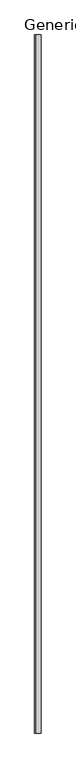
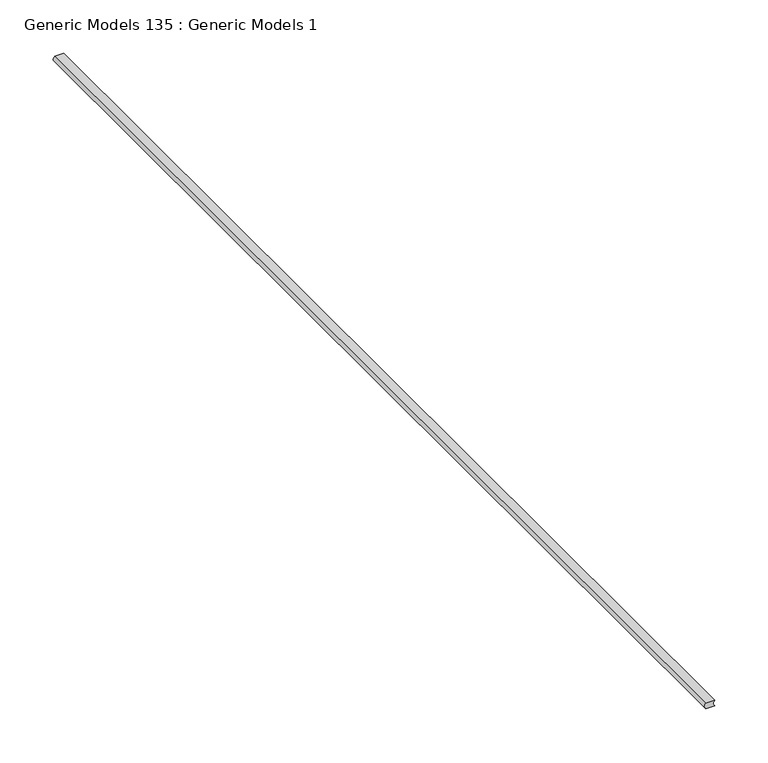
"""IFC4 building model written with IfcOpenShell, lengths in millimetres: proxy geometry, Generic Models 135 : Generic Models 1."""

import ifcopenshell
import ifcopenshell.guid

model = None  # the IFC model being written
_history = None  # IfcOwnerHistory: only IFC2X3 demands one
_inside = {}  # id of a spatial element -> (the spatial element, [elements in it])
_under = {}  # id of a project, library or spatial element -> (it, [spatial elements below it])
_declared = {}  # id of a project -> (the project, [libraries it declares])
_typed = {}  # id of a type object -> (the type object, [elements of that type])
_made_of = {}  # id of a material, layer set ... -> (it, [elements and type objects made of it])


def new_model(schema):
    """Start an empty IFC model of exactly this schema.

    Asked for "IFC4X3", IfcOpenShell would pick the latest addendum, in which some entities
    have other attributes; the version numbers below select the first issue.
    IFC2X3 requires an IfcOwnerHistory on every rooted entity: one is made here for all.
    """
    global model, _history
    if schema == "IFC4X3":
        model = ifcopenshell.file(schema_version=(4, 3, 0, 0))
    else:
        model = ifcopenshell.file(schema=schema)
    _inside.clear()
    _under.clear()
    _declared.clear()
    _typed.clear()
    _made_of.clear()
    _history = None
    if model.schema == "IFC2X3":
        org = make("IfcOrganization", Name="unknown")
        user = make(
            "IfcPersonAndOrganization",
            ThePerson=make("IfcPerson", FamilyName="unknown"),
            TheOrganization=org,
        )
        app = make(
            "IfcApplication",
            ApplicationDeveloper=org,
            Version="unknown",
            ApplicationFullName="unknown",
            ApplicationIdentifier="unknown",
        )
        _history = make(
            "IfcOwnerHistory",
            OwningUser=user,
            OwningApplication=app,
            ChangeAction="ADDED",
            CreationDate=0,
        )
    return model


def make(cls, **values):
    """One entity of the class cls with the attributes given. An attribute that is None is left unset."""
    return model.create_entity(
        cls, **{name: value for name, value in values.items() if value is not None}
    )


def rooted(cls, **values):
    """An entity with a GlobalId (a new one), such as an element, a storey or a relation."""
    return make(cls, GlobalId=ifcopenshell.guid.new(), OwnerHistory=_history, **values)


def si_unit(unit_type, name, prefix=None):
    """IfcSIUnit, for example si_unit("LENGTHUNIT", "METRE", prefix="MILLI")."""
    return make("IfcSIUnit", UnitType=unit_type, Prefix=prefix, Name=name)


def assignment(units):
    """IfcUnitAssignment: the units of a project."""
    return None if units is None else make("IfcUnitAssignment", Units=units)


def point(xyz):
    """IfcCartesianPoint."""
    return None if xyz is None else make("IfcCartesianPoint", Coordinates=xyz)


def direction(xyz):
    """IfcDirection."""
    return None if xyz is None else make("IfcDirection", DirectionRatios=xyz)


def frame(location, z_axis=None, x_axis=None):
    """IfcAxis2Placement3D, a coordinate frame: its origin and axes. An axis left out is left unset."""
    return make(
        "IfcAxis2Placement3D",
        Location=point(location),
        Axis=direction(z_axis),
        RefDirection=direction(x_axis),
    )


def frame_2d(location, x_axis=None):
    """IfcAxis2Placement2D, a coordinate frame in the plane: its origin and x axis."""
    return make(
        "IfcAxis2Placement2D", Location=point(location), RefDirection=direction(x_axis)
    )


def origin():
    """The frame at (0, 0, 0) with its axes left unset."""
    return frame((0.0, 0.0, 0.0))


def place(relative_to, where):
    """IfcLocalPlacement: puts the frame where relative to a parent placement (None: the world)."""
    return make(
        "IfcLocalPlacement", PlacementRelTo=relative_to, RelativePlacement=where
    )


def context(
    kind, dimensions, precision=None, world=None, true_north=None, identifier=None
):
    """IfcGeometricRepresentationContext, for example the 3D "Model" context."""
    return make(
        "IfcGeometricRepresentationContext",
        ContextIdentifier=identifier,
        ContextType=kind,
        CoordinateSpaceDimension=dimensions,
        Precision=precision,
        WorldCoordinateSystem=world,
        TrueNorth=true_north,
    )


def project(units=None, contexts=None):
    """IfcProject with its units and contexts."""
    return rooted(
        "IfcProject",
        Name="project",
        RepresentationContexts=contexts,
        UnitsInContext=assignment(units),
    )


def spatial(cls, under=None, at=None, **own):
    """A site, building, storey or space (cls), placed at a placement, below another one or the project."""
    s = rooted(cls, ObjectPlacement=at, **own)
    if under is not None:
        _under.setdefault(under.id(), (under, []))[1].append(s)
    return s


def polyline(points):
    """IfcPolyline through the points."""
    return make("IfcPolyline", Points=[point(p) for p in points])


def circle_curve(where, radius):
    """IfcCircle in the frame where."""
    return make("IfcCircle", Position=where, Radius=radius)


def trimmed(basis, trim1, trim2, sense, master):
    """IfcTrimmedCurve: the piece of a basis curve between two trims."""
    return make(
        "IfcTrimmedCurve",
        BasisCurve=basis,
        Trim1=trim1,
        Trim2=trim2,
        SenseAgreement=sense,
        MasterRepresentation=master,
    )


def segment(curve, same_sense, transition):
    """IfcCompositeCurveSegment."""
    return make(
        "IfcCompositeCurveSegment",
        Transition=transition,
        SameSense=same_sense,
        ParentCurve=curve,
    )


def composite_curve(segments, self_intersect=None):
    """IfcCompositeCurve: segments joined end to end."""
    return make("IfcCompositeCurve", Segments=segments, SelfIntersect=self_intersect)


def outline(outer, holes=None, kind="AREA"):
    """IfcArbitraryClosedProfileDef: a profile drawn as a closed curve; with holes, ...WithVoids."""
    if holes is None:
        return make("IfcArbitraryClosedProfileDef", ProfileType=kind, OuterCurve=outer)
    return make(
        "IfcArbitraryProfileDefWithVoids",
        ProfileType=kind,
        OuterCurve=outer,
        InnerCurves=holes,
    )


def extrude(swept, where, along, depth):
    """IfcExtrudedAreaSolid: the profile swept, set in the frame where, extruded along a direction by depth."""
    return make(
        "IfcExtrudedAreaSolid",
        SweptArea=swept,
        Position=where,
        ExtrudedDirection=direction(along),
        Depth=depth,
    )


def shape(context_of_items, identifier, shape_type, items):
    """IfcShapeRepresentation: the items that make up one representation, for example the "Body"."""
    return make(
        "IfcShapeRepresentation",
        ContextOfItems=context_of_items,
        RepresentationIdentifier=identifier,
        RepresentationType=shape_type,
        Items=items,
    )


def source(mapping_origin, context_of_items, identifier, shape_type, items):
    """IfcRepresentationMap: a shape defined once, which mapped items show again and again."""
    return make(
        "IfcRepresentationMap",
        MappingOrigin=mapping_origin,
        MappedRepresentation=shape(context_of_items, identifier, shape_type, items),
    )


def transform(
    local_origin,
    x_axis=None,
    y_axis=None,
    z_axis=None,
    scale=None,
    scale2=None,
    scale3=None,
    uniform=True,
):
    """IfcCartesianTransformationOperator3D, or its non-uniform kind. x_axis, y_axis, z_axis: its Axis1, 2, 3."""
    if uniform:
        return make(
            "IfcCartesianTransformationOperator3D",
            Axis1=direction(x_axis),
            Axis2=direction(y_axis),
            LocalOrigin=point(local_origin),
            Scale=scale,
            Axis3=direction(z_axis),
        )
    return make(
        "IfcCartesianTransformationOperator3DnonUniform",
        Axis1=direction(x_axis),
        Axis2=direction(y_axis),
        LocalOrigin=point(local_origin),
        Scale=scale,
        Axis3=direction(z_axis),
        Scale2=scale2,
        Scale3=scale3,
    )


def mapped(mapping_source, mapping_target):
    """IfcMappedItem: shows the shape of a source again, moved by a transform."""
    return make(
        "IfcMappedItem", MappingSource=mapping_source, MappingTarget=mapping_target
    )


def made_of(thing, what):
    """Note that an element or type object is made of a material, layer set ...; save() writes the relation."""
    if what is not None:
        _made_of.setdefault(what.id(), (what, []))[1].append(thing)
    return thing


def element(
    cls,
    number,
    at=None,
    inside=None,
    cuts=None,
    type_object=None,
    material=None,
    context=None,
    identifier="Body",
    shape_type=None,
    held_by="IfcProductDefinitionShape",
    body=None,
    shapes=None,
    **own,
):
    """One element of the class cls, such as IfcWall. Its Tag is "e" and its number.

    at: its placement. inside: the storey or other place that contains it. cuts: it is an
    opening in that element (IfcRelVoidsElement). A single representation is given by context,
    identifier, shape_type and body (its items); several are given by shapes. held_by: the class
    of the entity that holds the representations. save() writes the other relations.
    """
    e = rooted(cls, Tag="e%d" % number, ObjectPlacement=at, **own)
    if body is not None:
        shapes = [shape(context, identifier, shape_type, body)]
    if shapes is not None:
        e.Representation = make(held_by, Representations=shapes)
    if inside is not None:
        _inside.setdefault(inside.id(), (inside, []))[1].append(e)
    if cuts is not None:
        rooted(
            "IfcRelVoidsElement", RelatingBuildingElement=cuts, RelatedOpeningElement=e
        )
    if type_object is not None:
        _typed.setdefault(type_object.id(), (type_object, []))[1].append(e)
    return made_of(e, material)


def aggregate(whole, parts):
    """IfcRelAggregates: a whole, such as a stair, and the parts it consists of."""
    return rooted("IfcRelAggregates", RelatingObject=whole, RelatedObjects=parts)


def save(model, path):
    """Write the relations noted so far, then the file.

    IfcRelAggregates (storeys below a building ...), IfcRelContainedInSpatialStructure (elements
    in a storey), IfcRelDefinesByType, IfcRelAssociatesMaterial and IfcRelDeclares: one each for
    every whole, place, type object, material and project.
    """
    for whole, parts in _under.values():
        aggregate(whole, parts)
    for where, things in _inside.values():
        rooted(
            "IfcRelContainedInSpatialStructure",
            RelatedElements=things,
            RelatingStructure=where,
        )
    for kind, things in _typed.values():
        rooted("IfcRelDefinesByType", RelatedObjects=things, RelatingType=kind)
    for what, things in _made_of.values():
        rooted("IfcRelAssociatesMaterial", RelatedObjects=things, RelatingMaterial=what)
    for by, libraries in _declared.values():
        rooted("IfcRelDeclares", RelatingContext=by, RelatedDefinitions=libraries)
    model.write(path)


def generic_models_135_generic_models_1_f2b08089(model_context):
    return source(origin(), model_context, "Body", "SweptSolid", [
        extrude(outline(composite_curve([segment(trimmed(circle_curve(frame_2d((-222.801067, 48169.1006666)), 4.3100275), [point((-225.976067, 48166.1859261))], [point((-219.626067, 48166.1859261))], True, "CARTESIAN"), True, "CONTINUOUS"), segment(polyline([(-219.626067, 48166.1859261), (-219.626067, 48156.6609261)]), True, "CONTINUOUS"), segment(trimmed(circle_curve(frame_2d((-222.801067, 48159.5756666)), 4.3100275), [point((-219.626067, 48156.6609261))], [point((-225.976067, 48156.6609261))], False, "CARTESIAN"), True, "CONTINUOUS"), segment(polyline([(-225.976067, 48156.6609261), (-225.976067, 48166.1859261)]), True, "CONTINUOUS")], self_intersect=False)), frame((0.0, 0.0, 0.0), z_axis=(0.0, 1.0, 0.0), x_axis=(0.0, 0.0, 1.0)), (0.0, 0.0, 1.0), 1219.2),
    ])


if __name__ == "__main__":
    model = new_model("IFC4")
    model_context = context("Model", 3, world=origin())
    ifc_project = project(units=[si_unit("LENGTHUNIT", "METRE", prefix="MILLI")], contexts=[model_context])
    site = spatial("IfcSite", under=ifc_project)
    building = spatial("IfcBuilding", under=site)
    placement = place(None, origin())
    generic_models_135_generic_models_1_shape = generic_models_135_generic_models_1_f2b08089(model_context)
    element("IfcBuildingElementProxy", 1, Name="Generic Models 135 : Generic Models 1", ObjectType="Generic Models 135 : Generic Models 1", at=placement, inside=building, context=model_context, shape_type="MappedRepresentation", body=[
        mapped(generic_models_135_generic_models_1_shape, transform((0.0, 0.0, 0.0), x_axis=(1.0, 0.0, 0.0), y_axis=(0.0, 1.0, 0.0), z_axis=(0.0, 0.0, 1.0))),
    ])
    save(model, "model.ifc")

# Revit data of these elements
# Element 1 (IfcBuildingElementProxy, "Generic Models 135 : Generic Models 1")
#   Materials on its faces: "SEALANT (W/ BACKER ROD IF NECESSARY)"
# Materials
#   "SEALANT (W/ BACKER ROD IF NECESSARY)": class "Unassigned", colour RGB 120 120 120, transparency 0, Cost = 0
